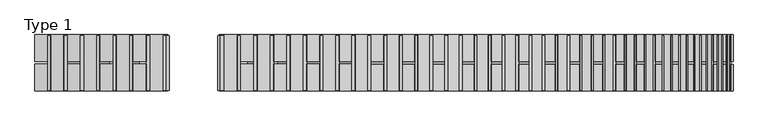
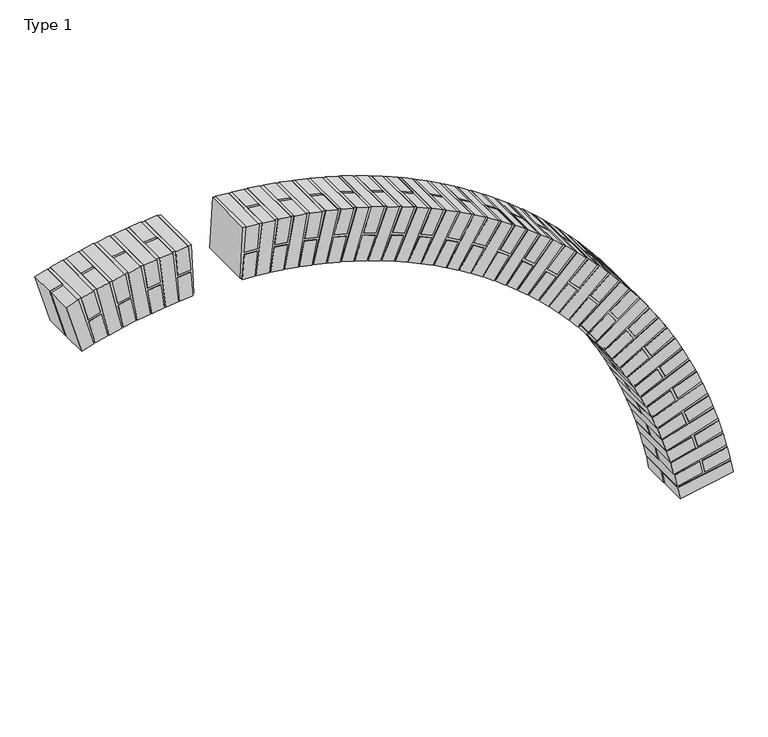
"""IFC4 building model written with IfcOpenShell, lengths in millimetres: proxy geometry, 00_GM_toog : Type 1."""

from ifc_helpers import new_model, si_unit, frame, origin, place, context, project, spatial, polyline, outline, extrude, source, transform, mapped, element, save


def type_1_09ec10ce(model_context):
    return source(origin(), model_context, "Body", "SweptSolid", [
        extrude(outline(polyline([(-51.3105527, 298.3168038), (-50.0324743, 286.1851231), (-149.0433825, 272.1551526), (-142.0283972, 222.6496985), (-43.0174891, 236.6796691), (-41.3072329, 224.6102198), (-244.0930868, 202.1502071), (-245.111966, 208.0426268), (-151.9800205, 221.2395409), (-158.9950058, 270.744995), (-252.3004379, 257.5234976), (-253.31442, 263.3875962), (-51.3105527, 298.3168038)])), frame((0.0, 2.5, 0.0), z_axis=(0.0, 1.0, 0.0), x_axis=(0.0, 0.0, 1.0)), (0.0, 0.0, 1.0), 205.0),
        extrude(outline(polyline([(0.0, 50.0), (210.0, 50.0), (210.0, 0.0), (0.0, 0.0), (0.0, 50.0)])), frame((222.6496985, 210.0, -142.0283972), z_axis=(0.14029970561810096, 0.0, 0.9901090811640273), x_axis=(0.0, -1.0, 0.0)), (0.0, 0.0, 1.0), 100.0),
        extrude(outline(polyline([(0.0, 49.9999999), (210.0, 49.9999999), (210.0, 0.0), (0.0, 0.0), (0.0, 49.9999999)])), frame((207.2095704, 210.0, -250.9909286), z_axis=(0.14029970561810096, 0.0, 0.9901090811640273), x_axis=(0.0, -1.0, 0.0)), (0.0, 0.0, 1.0), 100.0),
        extrude(outline(polyline([(210.0, 50.0), (210.0, 0.0), (110.0, 0.0), (110.0, 50.0), (210.0, 50.0)])), frame((311.8048021, 0.0, -266.7590939), z_axis=(0.17038513774279196, 0.0, 0.9853775443130262), x_axis=(0.0, 1.0, 0.0)), (0.0, 0.0, 1.0), 210.0),
        extrude(outline(polyline([(100.0, 50.0), (100.0, 0.0), (0.0, 0.0), (0.0, 50.0), (100.0, 50.0)])), frame((311.8048021, 0.0, -266.7590939), z_axis=(0.17038513774279196, 0.0, 0.9853775443130262), x_axis=(0.0, 1.0, 0.0)), (0.0, 0.0, 1.0), 210.0),
        extrude(outline(polyline([(-36.8943593, 174.8755374), (-36.357169, 162.6885531), (-136.0385268, 154.7119056), (-132.0502031, 104.8712267), (-32.3688453, 112.8478742), (-31.3964904, 100.696697), (-235.1735118, 90.6229563), (-235.8317995, 96.5664722), (-142.0692136, 104.0694909), (-146.0575373, 153.9101698), (-239.9947846, 146.3931745), (-240.6499084, 152.3081238), (-36.8943593, 174.8755374)])), frame((0.0, 2.5, 0.0), z_axis=(0.0, 1.0, 0.0), x_axis=(0.0, 0.0, 1.0)), (0.0, 0.0, 1.0), 205.0),
        extrude(outline(polyline([(0.0, 50.0), (210.0, 50.0), (210.0, 0.0), (0.0, 0.0), (0.0, 50.0)])), frame((104.8712267, 210.0, -132.0502031), z_axis=(0.07976647429823253, 0.0, 0.9968135781469017), x_axis=(0.0, -1.0, 0.0)), (0.0, 0.0, 1.0), 100.0),
        extrude(outline(polyline([(0.0, 50.0), (210.0, 50.0), (210.0, 0.0), (0.0, 0.0), (0.0, 50.0)])), frame((96.0928435, 210.0, -241.7505714), z_axis=(0.07976647429823253, 0.0, 0.9968135781469017), x_axis=(0.0, -1.0, 0.0)), (0.0, 0.0, 1.0), 100.0),
        extrude(outline(polyline([(210.0, 50.0), (210.0, 0.0), (110.0, 0.0), (110.0, 50.0), (210.0, 50.0)])), frame((201.453981, 0.0, -251.1222434), z_axis=(0.11008414261687069, 0.0, 0.9939222713795623), x_axis=(0.0, 1.0, 0.0)), (0.0, 0.0, 1.0), 210.0),
        extrude(outline(polyline([(100.0, 50.0), (100.0, 0.0), (0.0, 0.0), (0.0, 50.0), (100.0, 50.0)])), frame((201.453981, 0.0, -251.1222434), z_axis=(0.11008414261687069, 0.0, 0.9939222713795623), x_axis=(0.0, 1.0, 0.0)), (0.0, 0.0, 1.0), 210.0),
        extrude(outline(polyline([(-73.2145142, 420.6515468), (-71.2002884, 408.6201689), (-169.1734934, 388.5889155), (-159.1578667, 339.602313), (-61.1846617, 359.6335665), (-58.742848, 347.6906134), (-259.7853565, 312.9276379), (-261.161048, 318.747105), (-169.0051901, 337.5889643), (-179.0208168, 386.5755668), (-271.348343, 367.6986088), (-272.7174225, 373.4901055), (-73.2145142, 420.6515468)])), frame((0.0, 2.5, 0.0), z_axis=(0.0, 1.0, 0.0), x_axis=(0.0, 0.0, 1.0)), (0.0, 0.0, 1.0), 205.0),
        extrude(outline(polyline([(0.0, 50.0), (210.0, 50.0), (210.0, 0.0), (0.0, 0.0), (0.0, 50.0)])), frame((339.602313, 210.0, -159.1578667), z_axis=(0.20031253413085065, 0.0, 0.9797320494247787), x_axis=(0.0, -1.0, 0.0)), (0.0, 0.0, 1.0), 100.0),
        extrude(outline(polyline([(0.0, 49.9999999), (210.0, 49.9999999), (210.0, 0.0), (0.0, 0.0), (0.0, 49.9999999)])), frame((317.5577109, 210.0, -266.978395), z_axis=(0.20031253413085065, 0.0, 0.9797320494247787), x_axis=(0.0, -1.0, 0.0)), (0.0, 0.0, 1.0), 100.0),
        extrude(outline(polyline([(210.0, 50.0), (210.0, 0.0), (110.0, 0.0), (110.0, 50.0), (210.0, 50.0)])), frame((420.9990698, 0.0, -289.084566), z_axis=(0.2300541365036329, 0.0, 0.973177832812466), x_axis=(0.0, 1.0, 0.0)), (0.0, 0.0, 1.0), 210.0),
        extrude(outline(polyline([(100.0, 50.0), (100.0, 0.0), (0.0, 0.0), (0.0, 50.0), (100.0, 50.0)])), frame((420.9990698, 0.0, -289.084566), z_axis=(0.2300541365036329, 0.0, 0.973177832812466), x_axis=(0.0, 1.0, 0.0)), (0.0, 0.0, 1.0), 210.0),
        extrude(outline(polyline([(-102.5249972, 541.4259997), (-99.7820951, 529.5395517), (-196.3541925, 503.5813158), (-183.3750746, 455.2952671), (-86.8029772, 481.253503), (-83.6386631, 469.4813452), (-282.1921149, 422.5443504), (-283.9195159, 428.2692793), (-193.0815721, 452.6861951), (-206.06069, 500.9722438), (-297.0678472, 476.509844), (-298.7869457, 482.2072569), (-102.5249972, 541.4259997)])), frame((0.0, 2.5, 0.0), z_axis=(0.0, 1.0, 0.0), x_axis=(0.0, 0.0, 1.0)), (0.0, 0.0, 1.0), 205.0),
        extrude(outline(polyline([(0.0, 50.0), (210.0, 50.0), (210.0, 0.0), (0.0, 0.0), (0.0, 50.0)])), frame((455.2952671, 210.0, -183.3750746), z_axis=(0.2595823589102464, 0.0, 0.9657209736474569), x_axis=(0.0, -1.0, 0.0)), (0.0, 0.0, 1.0), 100.0),
        extrude(outline(polyline([(0.0, 50.0), (210.0, 50.0), (210.0, 0.0), (0.0, 0.0), (0.0, 50.0)])), frame((426.7279592, 210.0, -289.6536695), z_axis=(0.2595823589102464, 0.0, 0.9657209736474569), x_axis=(0.0, -1.0, 0.0)), (0.0, 0.0, 1.0), 100.0),
        extrude(outline(polyline([(210.0, 50.0000001), (210.0, 0.0), (110.0, 0.0), (110.0, 50.0000001), (210.0, 50.0000001)])), frame((528.6317584, 0.0, -318.0158494), z_axis=(0.28886981331416434, 0.0, 0.9573683883207341), x_axis=(0.0, 1.0, 0.0)), (0.0, 0.0, 1.0), 210.0),
        extrude(outline(polyline([(100.0, 50.0000001), (100.0, 0.0), (0.0, 0.0), (0.0, 50.0000001), (100.0, 50.0000001)])), frame((528.6317584, 0.0, -318.0158494), z_axis=(0.28886981331416434, 0.0, 0.9573683883207341), x_axis=(0.0, 1.0, 0.0)), (0.0, 0.0, 1.0), 210.0),
        extrude(outline(polyline([(-139.1332824, 660.1921832), (-135.6718782, 648.4947544), (-230.4846606, 616.7058209), (-214.5901938, 569.2994297), (-119.7774114, 601.0883632), (-115.9023342, 589.5306663), (-311.2302503, 530.593752), (-313.3029535, 536.2029076), (-224.119862, 566.1043122), (-240.0143287, 613.5107034), (-329.3635509, 583.5535983), (-331.426292, 589.1357943), (-139.1332824, 660.1921832)])), frame((0.0, 2.5, 0.0), z_axis=(0.0, 1.0, 0.0), x_axis=(0.0, 0.0, 1.0)), (0.0, 0.0, 1.0), 205.0),
        extrude(outline(polyline([(0.0, 50.0), (210.0, 50.0), (210.0, 0.0), (0.0, 0.0), (0.0, 50.0)])), frame((569.2994297, 210.0, -214.5901938), z_axis=(0.3178893349961213, 0.0, 0.9481278240278174), x_axis=(0.0, -1.0, 0.0)), (0.0, 0.0, 1.0), 100.0),
        extrude(outline(polyline([(0.0, 50.0), (210.0, 50.0), (210.0, 0.0), (0.0, 0.0), (0.0, 50.0)])), frame((534.3153787, 210.0, -318.9326444), z_axis=(0.3178893349961213, 0.0, 0.9481278240278174), x_axis=(0.0, -1.0, 0.0)), (0.0, 0.0, 1.0), 100.0),
        extrude(outline(polyline([(210.0, 50.0), (210.0, 0.0), (110.0, 0.0), (110.0, 50.0), (210.0, 50.0)])), frame((634.3036342, 0.0, -353.4456316), z_axis=(0.3466140077500296, 0.0, 0.9380078515830571), x_axis=(0.0, 1.0, 0.0)), (0.0, 0.0, 1.0), 210.0),
        extrude(outline(polyline([(100.0, 50.0), (100.0, 0.0), (0.0, 0.0), (0.0, 50.0), (100.0, 50.0)])), frame((634.3036342, 0.0, -353.4456316), z_axis=(0.3466140077500296, 0.0, 0.9380078515830571), x_axis=(0.0, 1.0, 0.0)), (0.0, 0.0, 1.0), 210.0),
        extrude(outline(polyline([(-182.9035816, 776.5095671), (-178.7365144, 765.0445459), (-271.4383001, 727.5428271), (-252.6874407, 681.1919342), (-159.9856549, 718.6936531), (-155.414188, 707.3932871), (-346.7920539, 636.6750634), (-349.2023711, 642.14764), (-262.0049317, 677.4226224), (-280.7557912, 723.7735153), (-368.1156623, 688.4328225), (-370.5143948, 693.8790961), (-182.9035816, 776.5095671)])), frame((0.0, 2.5, 0.0), z_axis=(0.0, 1.0, 0.0), x_axis=(0.0, 0.0, 1.0)), (0.0, 0.0, 1.0), 205.0),
        extrude(outline(polyline([(0.0, 50.0), (210.0, 50.0), (210.0, 0.0), (0.0, 0.0), (0.0, 50.0)])), frame((681.1919342, 210.0, -252.6874407), z_axis=(0.37501718884823365, 0.0, 0.9270178574700534), x_axis=(0.0, -1.0, 0.0)), (0.0, 0.0, 1.0), 100.0),
        extrude(outline(polyline([(0.0, 50.0), (210.0, 50.0), (210.0, 0.0), (0.0, 0.0), (0.0, 50.0)])), frame((639.9209035, 210.0, -354.7067175), z_axis=(0.37501718884823365, 0.0, 0.9270178574700534), x_axis=(0.0, -1.0, 0.0)), (0.0, 0.0, 1.0), 100.0),
        extrude(outline(polyline([(210.0, 50.0), (210.0, 0.0), (110.0, 0.0), (110.0, 50.0), (210.0, 50.0)])), frame((737.6227368, 0.0, -395.2424957), z_axis=(0.40307253375327073, 0.0, 0.9151680351354708), x_axis=(0.0, 1.0, 0.0)), (0.0, 0.0, 1.0), 210.0),
        extrude(outline(polyline([(100.0, 50.0), (100.0, 0.0), (0.0, 0.0), (0.0, 50.0), (100.0, 50.0)])), frame((737.6227368, 0.0, -395.2424957), z_axis=(0.40307253375327073, 0.0, 0.9151680351354708), x_axis=(0.0, 1.0, 0.0)), (0.0, 0.0, 1.0), 210.0),
        extrude(outline(polyline([(-233.6735411, 889.9467043), (-228.8162674, 878.7566171), (-319.0632049, 835.6812151), (-297.5255039, 790.5577463), (-207.2785664, 833.6331483), (-202.0276663, 822.6320289), (-388.7456188, 740.3948054), (-391.4846098, 745.7105041), (-306.5962573, 786.2282216), (-328.1339583, 831.3516903), (-413.1804412, 790.7584963), (-415.9062676, 796.048646), (-233.6735411, 889.9467043)])), frame((0.0, 2.5, 0.0), z_axis=(0.0, 1.0, 0.0), x_axis=(0.0, 0.0, 1.0)), (0.0, 0.0, 1.0), 205.0),
        extrude(outline(polyline([(0.0, 50.0), (210.0, 50.0), (210.0, 0.0), (0.0, 0.0), (0.0, 50.0)])), frame((790.5577463, 210.0, -297.5255039), z_axis=(0.43075402055290246, 0.0, 0.9024693755344331), x_axis=(0.0, -1.0, 0.0)), (0.0, 0.0, 1.0), 100.0),
        extrude(outline(polyline([(0.0, 50.0), (210.0, 50.0), (210.0, 0.0), (0.0, 0.0), (0.0, 50.0)])), frame((743.1528195, 210.0, -396.8431948), z_axis=(0.43075402055290246, 0.0, 0.9024693755344331), x_axis=(0.0, -1.0, 0.0)), (0.0, 0.0, 1.0), 100.0),
        extrude(outline(polyline([(210.0, 50.0), (210.0, 0.0), (110.0, 0.0), (110.0, 50.0), (210.0, 50.0)])), frame((838.2058326, 0.0, -443.2514078), z_axis=(0.458035974096042, 0.0, 0.8889336569361574), x_axis=(0.0, 1.0, 0.0)), (0.0, 0.0, 1.0), 210.0),
        extrude(outline(polyline([(100.0, 50.0), (100.0, 0.0), (0.0, 0.0), (0.0, 50.0), (100.0, 50.0)])), frame((838.2058326, 0.0, -443.2514078), z_axis=(0.458035974096042, 0.0, 0.8889336569361574), x_axis=(0.0, 1.0, 0.0)), (0.0, 0.0, 1.0), 210.0),
        extrude(outline(polyline([(-291.2548438, 1000.0828313), (-285.7253803, 989.2091846), (-373.1827237, 940.7198756), (-348.9380692, 896.9912039), (-261.4807258, 945.4805129), (-255.5698695, 934.8194455), (-436.9353302, 841.3682584), (-439.9928353, 846.5073621), (-357.7284394, 892.1175254), (-381.9730939, 935.8461971), (-464.3907322, 890.151071), (-467.4335419, 895.2654744), (-291.2548438, 1000.0828313)])), frame((0.0, 2.5, 0.0), z_axis=(0.0, 1.0, 0.0), x_axis=(0.0, 0.0, 1.0)), (0.0, 0.0, 1.0), 205.0),
        extrude(outline(polyline([(0.0, 50.0), (210.0, 50.0), (210.0, 0.0), (0.0, 0.0), (0.0, 50.0)])), frame((896.9912039, 210.0, -348.9380692), z_axis=(0.4848930898069246, 0.0, 0.8745734339993948), x_axis=(0.0, -1.0, 0.0)), (0.0, 0.0, 1.0), 100.0),
        extrude(outline(polyline([(0.0, 50.0), (210.0, 50.0), (210.0, 0.0), (0.0, 0.0), (0.0, 50.0)])), frame((843.6282164, 210.0, -445.1857828), z_axis=(0.4848930898069246, 0.0, 0.8745734339993948), x_axis=(0.0, -1.0, 0.0)), (0.0, 0.0, 1.0), 100.0),
        extrude(outline(polyline([(210.0, 50.0), (210.0, 0.0), (110.0, 0.0), (110.0, 50.0), (210.0, 50.0)])), frame((935.6798366, 0.0, -497.2942922), z_axis=(0.5113004571556836, 0.0, 0.8594020261276959), x_axis=(0.0, 1.0, 0.0)), (0.0, 0.0, 1.0), 210.0),
        extrude(outline(polyline([(100.0, 50.0), (100.0, 0.0), (0.0, 0.0), (0.0, 50.0), (100.0, 50.0)])), frame((935.6798366, 0.0, -497.2942922), z_axis=(0.5113004571556836, 0.0, 0.8594020261276959), x_axis=(0.0, 1.0, 0.0)), (0.0, 0.0, 1.0), 210.0),
        extrude(outline(polyline([(-355.4339079, 1106.5094287), (-349.2527645, 1095.9925552), (-433.5961151, 1042.2691969), (-406.7344359, 1000.0975217), (-322.3910854, 1053.82088), (-315.8421974, 1043.5394089), (-491.1824416, 939.2208894), (-494.5471198, 944.1643361), (-415.2118175, 994.6977669), (-442.0734967, 1036.8694422), (-521.5565851, 986.2418775), (-524.9050916, 991.1615642), (-355.4339079, 1106.5094287)])), frame((0.0, 2.5, 0.0), z_axis=(0.0, 1.0, 0.0), x_axis=(0.0, 0.0, 1.0)), (0.0, 0.0, 1.0), 205.0),
        extrude(outline(polyline([(0.0, 50.0), (210.0, 50.0), (210.0, 0.0), (0.0, 0.0), (0.0, 50.0)])), frame((1000.0975217, 210.0, -406.7344359), z_axis=(0.5372335827633249, 0.0, 0.8434335051154191), x_axis=(0.0, -1.0, 0.0)), (0.0, 0.0, 1.0), 100.0),
        extrude(outline(polyline([(0.0, 50.0), (210.0, 50.0), (210.0, 0.0), (0.0, 0.0), (0.0, 50.0)])), frame((940.9744086, 210.0, -499.5551681), z_axis=(0.5372335827633249, 0.0, 0.8434335051154191), x_axis=(0.0, -1.0, 0.0)), (0.0, 0.0, 1.0), 100.0),
        extrude(outline(polyline([(210.0, 50.0), (210.0, 0.0), (110.0, 0.0), (110.0, 50.0), (210.0, 50.0)])), frame((1029.683196, 0.0, -557.1706918), z_axis=(0.562668413119899, 0.0, 0.8266826820958176), x_axis=(0.0, 1.0, 0.0)), (0.0, 0.0, 1.0), 210.0),
        extrude(outline(polyline([(100.0, 50.0), (100.0, 0.0), (0.0, 0.0), (0.0, 50.0), (100.0, 50.0)])), frame((1029.683196, 0.0, -557.1706918), z_axis=(0.562668413119899, 0.0, 0.8266826820958176), x_axis=(0.0, 1.0, 0.0)), (0.0, 0.0, 1.0), 210.0),
        extrude(outline(polyline([(-425.9726788, 1208.8317365), (-419.162783, 1198.7106457), (-500.0792923, 1139.9525101), (-470.7002245, 1099.4942554), (-389.7837151, 1158.252391), (-382.6210868, 1148.3886526), (-551.2857383, 1033.5897414), (-554.9451095, 1038.3191945), (-478.833173, 1093.5884532), (-508.2122409, 1134.0467079), (-584.4659589, 1078.6744934), (-588.1077418, 1083.3812152), (-425.9726788, 1208.8317365)])), frame((0.0, 2.5, 0.0), z_axis=(0.0, 1.0, 0.0), x_axis=(0.0, 0.0, 1.0)), (0.0, 0.0, 1.0), 205.0),
        extrude(outline(polyline([(0.0, 50.0), (210.0, 50.0), (210.0, 0.0), (0.0, 0.0), (0.0, 50.0)])), frame((1099.4942554, 210.0, -470.7002245), z_axis=(0.587581356894572, 0.0, 0.8091650938034423), x_axis=(0.0, -1.0, 0.0)), (0.0, 0.0, 1.0), 100.0),
        extrude(outline(polyline([(0.0, 50.0), (210.0, 50.0), (210.0, 0.0), (0.0, 0.0), (0.0, 50.0)])), frame((1034.8303175, 210.0, -559.7496824), z_axis=(0.587581356894572, 0.0, 0.8091650938034423), x_axis=(0.0, -1.0, 0.0)), (0.0, 0.0, 1.0), 100.0),
        extrude(outline(polyline([(210.0, 50.0), (210.0, 0.0), (110.0, 0.0), (110.0, 50.0), (210.0, 50.0)])), frame((1119.8672315, 0.0, -622.6585117), z_axis=(0.6119493068171298, 0.0, 0.7908969881634614), x_axis=(0.0, 1.0, 0.0)), (0.0, 0.0, 1.0), 210.0),
        extrude(outline(polyline([(100.0, 50.0), (100.0, 0.0), (0.0, 0.0), (0.0, 50.0), (100.0, 50.0)])), frame((1119.8672315, 0.0, -622.6585117), z_axis=(0.6119493068171298, 0.0, 0.7908969881634614), x_axis=(0.0, 1.0, 0.0)), (0.0, 0.0, 1.0), 210.0),
        extrude(outline(polyline([(-502.6095127, 1306.6702186), (-495.1961237, 1296.9824519), (-572.3856546, 1233.4074858), (-540.5981716, 1194.8127203), (-463.4086406, 1258.3876865), (-455.6588397, 1248.9782674), (-617.022284, 1124.1247791), (-620.9627746, 1128.6226962), (-548.3565201, 1188.4227768), (-580.1440032, 1227.0175422), (-652.8855088, 1167.1060659), (-656.80706, 1171.5823645), (-502.6095127, 1306.6702186)])), frame((0.0, 2.5, 0.0), z_axis=(0.0, 1.0, 0.0), x_axis=(0.0, 0.0, 1.0)), (0.0, 0.0, 1.0), 205.0),
        extrude(outline(polyline([(0.0, 50.0), (210.0, 50.0), (210.0, 0.0), (0.0, 0.0), (0.0, 50.0)])), frame((1194.8127203, 210.0, -540.5981716), z_axis=(0.6357496611103878, 0.0, 0.771895309221417), x_axis=(0.0, -1.0, 0.0)), (0.0, 0.0, 1.0), 100.0),
        extrude(outline(polyline([(0.0, 50.0), (210.0, 50.0), (210.0, 0.0), (0.0, 0.0), (0.0, 50.0)])), frame((1124.8478107, 210.0, -625.546051), z_axis=(0.6357496611103878, 0.0, 0.771895309221417), x_axis=(0.0, -1.0, 0.0)), (0.0, 0.0, 1.0), 100.0),
        extrude(outline(polyline([(210.0, 50.0), (210.0, 0.0), (110.0, 0.0), (110.0, 50.0), (210.0, 50.0)])), frame((1205.8974304, 0.0, -693.514843), z_axis=(0.658960344453872, 0.0, 0.752177681427224), x_axis=(0.0, 1.0, 0.0)), (0.0, 0.0, 1.0), 210.0),
        extrude(outline(polyline([(100.0, 50.0), (100.0, 0.0), (0.0, 0.0), (0.0, 50.0), (100.0, 50.0)])), frame((1205.8974304, 0.0, -693.514843), z_axis=(0.658960344453872, 0.0, 0.752177681427224), x_axis=(0.0, 1.0, 0.0)), (0.0, 0.0, 1.0), 210.0),
        extrude(outline(polyline([(-585.0601464, 1399.6619703), (-577.0707622, 1390.4434618), (-650.2470015, 1322.2874789), (-616.1690101, 1285.6993592), (-542.9927708, 1353.8553421), (-534.684543, 1344.9351441), (-688.1482472, 1210.490188), (-692.355241, 1214.7398854), (-623.5239812, 1278.848976), (-657.6019727, 1315.4370957), (-726.5614515, 1251.2085824), (-730.7482251, 1255.4378542), (-585.0601464, 1399.6619703)])), frame((0.0, 2.5, 0.0), z_axis=(0.0, 1.0, 0.0), x_axis=(0.0, 0.0, 1.0)), (0.0, 0.0, 1.0), 205.0),
        extrude(outline(polyline([(0.0, 50.0), (210.0, 50.0), (210.0, 0.0), (0.0, 0.0), (0.0, 50.0)])), frame((1285.6993592, 210.0, -616.1690101), z_axis=(0.6815598284590672, 0.0, 0.7317623932881814), x_axis=(0.0, -1.0, 0.0)), (0.0, 0.0, 1.0), 100.0),
        extrude(outline(polyline([(0.0, 50.0), (210.0, 50.0), (210.0, 0.0), (0.0, 0.0), (0.0, 50.0)])), frame((1210.6929931, 210.0, -696.7002206), z_axis=(0.6815598284590672, 0.0, 0.7317623932881814), x_axis=(0.0, -1.0, 0.0)), (0.0, 0.0, 1.0), 100.0),
        extrude(outline(polyline([(210.0, 50.0), (210.0, 0.0), (110.0, 0.0), (110.0, 50.0), (210.0, 50.0)])), frame((1287.4546875, 0.0, -769.4768639), z_axis=(0.7035271516375073, 0.0, 0.7106683804059498), x_axis=(0.0, 1.0, 0.0)), (0.0, 0.0, 1.0), 210.0),
        extrude(outline(polyline([(100.0, 50.0), (100.0, 0.0), (0.0, 0.0), (0.0, 50.0), (100.0, 50.0)])), frame((1287.4546875, 0.0, -769.4768639), z_axis=(0.7035271516375073, 0.0, 0.7106683804059498), x_axis=(0.0, 1.0, 0.0)), (0.0, 0.0, 1.0), 210.0),
        extrude(outline(polyline([(-673.0187522, 1487.4620645), (-664.4830073, 1478.7470076), (-733.374528, 1406.2628137), (-697.1324311, 1371.8170533), (-628.2409103, 1444.3012472), (-619.4050728, 1435.9033572), (-764.3998058, 1292.3656196), (-768.8576982, 1296.3513341), (-704.0567436, 1364.53164), (-740.2988405, 1398.9774004), (-805.2205066, 1330.670088), (-809.6569728, 1334.6366457), (-673.0187522, 1487.4620645)])), frame((0.0, 2.5, 0.0), z_axis=(0.0, 1.0, 0.0), x_axis=(0.0, 0.0, 1.0)), (0.0, 0.0, 1.0), 205.0),
        extrude(outline(polyline([(0.0, 99.9999999), (210.0, 99.9999999), (210.0, 0.0), (0.0, 0.0), (0.0, 99.9999999)])), frame((1406.2628137, 210.0, -733.374528), z_axis=(-0.6889152079134424, 0.0, 0.7248419388429304), x_axis=(0.0, -1.0, 0.0)), (0.0, 0.0, 1.0), 50.0),
        extrude(outline(polyline([(0.0, 100.0), (210.0, 100.0), (210.0, 0.0), (0.0, 0.0), (0.0, 100.0)])), frame((1326.4932065, 210.0, -809.1903613), z_axis=(-0.6889152079134424, 0.0, 0.7248419388429304), x_axis=(0.0, -1.0, 0.0)), (0.0, 0.0, 1.0), 50.0),
        extrude(outline(polyline([(0.0, 100.0), (209.9999999, 100.0), (209.9999999, 0.0), (0.0, 0.0), (0.0, 100.0)])), frame((1364.2364889, 110.0, -850.2628142), z_axis=(-0.6665230523277088, 0.0, 0.7454844201697004), x_axis=(0.7454844201697004, 0.0, 0.6665230523277088)), (0.0, 0.0, 1.0), 50.0),
        extrude(outline(polyline([(0.0, 100.0), (209.9999999, 100.0), (209.9999999, 0.0), (0.0, 0.0), (0.0, 100.0)])), frame((1364.2364889, 0.0, -850.2628142), z_axis=(-0.6665230523277088, 0.0, 0.7454844201697004), x_axis=(0.7454844201697004, 0.0, 0.6665230523277088)), (0.0, 0.0, 1.0), 50.0),
        extrude(outline(polyline([(-766.1590722, 1569.7448312), (-757.1086274, 1561.565552), (-821.4598957, 1485.022007), (-783.1881232, 1452.8463729), (-718.8368549, 1529.3899178), (-709.5061817, 1521.5454855), (-845.4941258, 1369.4473798), (-850.1863815, 1373.1543275), (-789.6560932, 1445.1529526), (-827.9278656, 1477.3285868), (-888.57091, 1405.1958423), (-893.2406131, 1408.8849732), (-766.1590722, 1569.7448312)])), frame((0.0, 2.5, 0.0), z_axis=(0.0, 1.0, 0.0), x_axis=(0.0, 0.0, 1.0)), (0.0, 0.0, 1.0), 205.0),
        extrude(outline(polyline([(0.0, 100.0000001), (210.0, 100.0000001), (210.0, 0.0), (0.0, 0.0), (0.0, 100.0000001)])), frame((1485.022007, 210.0, -821.4598957), z_axis=(-0.643512682835849, 0.0, 0.7654354492897545), x_axis=(0.0, -1.0, 0.0)), (0.0, 0.0, 1.0), 50.0),
        extrude(outline(polyline([(0.0, 100.0), (210.0, 100.0), (210.0, 0.0), (0.0, 0.0), (0.0, 100.0)])), frame((1400.7850419, 210.0, -892.2791339), z_axis=(-0.643512682835849, 0.0, 0.7654354492897545), x_axis=(0.0, -1.0, 0.0)), (0.0, 0.0, 1.0), 50.0),
        extrude(outline(polyline([(0.0, 100.0), (210.0, 100.0), (210.0, 0.0), (0.0, 0.0), (0.0, 100.0)])), frame((1435.9580338, 110.0, -935.5730411), z_axis=(-0.6199054420311093, 0.0, 0.7846765212112665), x_axis=(0.7846765212112665, 0.0, 0.6199054420311093)), (0.0, 0.0, 1.0), 50.0),
        extrude(outline(polyline([(0.0, 100.0), (210.0, 100.0), (210.0, 0.0), (0.0, 0.0), (0.0, 100.0)])), frame((1435.9580338, 0.0, -935.5730411), z_axis=(-0.6199054420311093, 0.0, 0.7846765212112665), x_axis=(0.7846765212112665, 0.0, 0.6199054420311093)), (0.0, 0.0, 1.0), 50.0),
        extrude(outline(polyline([(-864.1356281, 1646.2050652), (-854.6040536, 1638.5919024), (-914.1763762, 1558.2729235), (-874.0168867, 1528.4867622), (-814.4445641, 1608.8057411), (-804.6536647, 1601.5438633), (-931.1304104, 1441.4495551), (-936.0396247, 1444.8639862), (-880.0045231, 1520.4138717), (-920.1640125, 1550.200033), (-976.3034966, 1474.5094128), (-981.1891156, 1477.9074329), (-864.1356281, 1646.2050652)])), frame((0.0, 2.5, 0.0), z_axis=(0.0, 1.0, 0.0), x_axis=(0.0, 0.0, 1.0)), (0.0, 0.0, 1.0), 205.0),
        extrude(outline(polyline([(0.0, 100.0), (210.0, 100.0), (210.0, 0.0), (0.0, 0.0), (0.0, 100.0)])), frame((1558.2729235, 210.0, -914.1763762), z_axis=(-0.5957232261172445, 0.0, 0.8031897894423599), x_axis=(0.0, -1.0, 0.0)), (0.0, 0.0, 1.0), 50.0),
        extrude(outline(polyline([(0.0, 100.0), (210.0, 100.0), (210.0, 0.0), (0.0, 0.0), (0.0, 100.0)])), frame((1469.881054, 210.0, -979.7363351), z_axis=(-0.5957232261172445, 0.0, 0.8031897894423599), x_axis=(0.0, -1.0, 0.0)), (0.0, 0.0, 1.0), 50.0),
        extrude(outline(polyline([(0.0, 100.0), (210.0, 100.0), (210.0, 0.0), (0.0, 0.0), (0.0, 100.0)])), frame((1502.3532911, 110.0, -1025.0911098), z_axis=(-0.5709884645992758, 0.0, 0.8209580825441465), x_axis=(0.8209580825441465, 0.0, 0.5709884645992758)), (0.0, 0.0, 1.0), 50.0),
        extrude(outline(polyline([(0.0, 100.0), (210.0, 100.0), (210.0, 0.0), (0.0, 0.0), (0.0, 100.0)])), frame((1502.3532911, 0.0, -1025.0911098), z_axis=(-0.5709884645992758, 0.0, 0.8209580825441465), x_axis=(0.8209580825441465, 0.0, 0.5709884645992758)), (0.0, 0.0, 1.0), 50.0),
        extrude(outline(polyline([(-966.5850031, 1716.5591585), (-956.6076536, 1709.5403512), (-1011.1800635, 1625.7438592), (-969.2818175, 1598.4576542), (-914.7094076, 1682.2541462), (-904.4945987, 1675.6017587), (-1020.9910156, 1508.1050735), (-1026.0989792, 1511.214323), (-974.7669108, 1590.0352375), (-1016.6651568, 1617.3214425), (-1068.0928468, 1538.3537), (-1073.1762598, 1541.4480054), (-966.5850031, 1716.5591585)])), frame((0.0, 2.5, 0.0), z_axis=(0.0, 1.0, 0.0), x_axis=(0.0, 0.0, 1.0)), (0.0, 0.0, 1.0), 205.0),
        extrude(outline(polyline([(0.0, 100.0), (210.0, 100.0), (210.0, 0.0), (0.0, 0.0), (0.0, 100.0)])), frame((1625.7438592, 210.0, -1011.1800635), z_axis=(-0.5457240994797231, 0.0, 0.8379649200575435), x_axis=(0.0, -1.0, 0.0)), (0.0, 0.0, 1.0), 50.0),
        extrude(outline(polyline([(0.0, 100.0), (210.0, 100.0), (210.0, 0.0), (0.0, 0.0), (0.0, 100.0)])), frame((1533.5249505, 210.0, -1071.2375667), z_axis=(-0.5457240994797231, 0.0, 0.8379649200575435), x_axis=(0.0, -1.0, 0.0)), (0.0, 0.0, 1.0), 50.0),
        extrude(outline(polyline([(0.0, 100.0), (210.0, 100.0), (210.0, 0.0), (0.0, 0.0), (0.0, 100.0)])), frame((1563.1759859, 110.0, -1118.4849779), z_axis=(-0.5199535639793587, 0.0, 0.854194527789287), x_axis=(0.854194527789287, 0.0, 0.5199535639793587)), (0.0, 0.0, 1.0), 50.0),
        extrude(outline(polyline([(0.0, 100.0), (210.0, 100.0), (210.0, 0.0), (0.0, 0.0), (0.0, 100.0)])), frame((1563.1759859, 0.0, -1118.4849779), z_axis=(-0.5199535639793587, 0.0, 0.854194527789287), x_axis=(0.854194527789287, 0.0, 0.5199535639793587)), (0.0, 0.0, 1.0), 50.0),
        extrude(outline(polyline([(-1073.1271897, 1780.5461522), (-1062.7410734, 1774.1477346), (-1112.1111495, 1687.1845493), (-1068.6295568, 1662.4995113), (-1019.2594808, 1749.4626965), (-1008.6586513, 1743.4444745), (-1114.7426284, 1569.1666948), (-1120.0303947, 1571.9592298), (-1073.5917616, 1653.7588091), (-1117.0733542, 1678.4438472), (-1163.5984934, 1596.4918913), (-1168.8608449, 1599.2710044), (-1073.1271897, 1780.5461522)])), frame((0.0, 2.5, 0.0), z_axis=(0.0, 1.0, 0.0), x_axis=(0.0, 0.0, 1.0)), (0.0, 0.0, 1.0), 205.0),
        extrude(outline(polyline([(0.0, 100.0000001), (210.0, 100.0000001), (210.0, 0.0), (0.0, 0.0), (0.0, 100.0000001)])), frame((1687.1845493, 210.0, -1112.1111495), z_axis=(-0.4937007608024789, 0.0, 0.8696318524427756), x_axis=(0.0, -1.0, 0.0)), (0.0, 0.0, 1.0), 50.0),
        extrude(outline(polyline([(0.0, 100.0000001), (210.0, 100.0000001), (210.0, 0.0), (0.0, 0.0), (0.0, 100.0000001)])), frame((1591.4806619, 210.0, -1166.4434303), z_axis=(-0.4937007608024789, 0.0, 0.8696318524427756), x_axis=(0.0, -1.0, 0.0)), (0.0, 0.0, 1.0), 50.0),
        extrude(outline(polyline([(0.0, 100.0), (210.0, 100.0), (210.0, 0.0), (0.0, 0.0), (0.0, 100.0)])), frame((1618.2005133, 110.0, -1215.4082269), z_axis=(-0.46699003996658267, 0.0, 0.8842625755803587), x_axis=(0.8842625755803587, 0.0, 0.46699003996658267)), (0.0, 0.0, 1.0), 50.0),
        extrude(outline(polyline([(0.0, 100.0), (210.0, 100.0), (210.0, 0.0), (0.0, 0.0), (0.0, 100.0)])), frame((1618.2005133, 0.0, -1215.4082269), z_axis=(-0.46699003996658267, 0.0, 0.8842625755803587), x_axis=(0.8842625755803587, 0.0, 0.46699003996658267)), (0.0, 0.0, 1.0), 50.0),
        extrude(outline(polyline([(-1183.3669992, 1837.9287043), (-1172.6106405, 1832.1744095), (-1216.5952582, 1742.3670968), (-1171.6916018, 1720.374788), (-1127.7069842, 1810.1821007), (-1116.7594551, 1804.8203672), (-1212.0375032, 1624.4079279), (-1217.4854587, 1626.8733903), (-1176.1125121, 1711.3482215), (-1221.0161685, 1733.3405303), (-1262.4661848, 1648.7083391), (-1267.8879555, 1651.1619516), (-1183.3669992, 1837.9287043)])), frame((0.0, 2.5, 0.0), z_axis=(0.0, 1.0, 0.0), x_axis=(0.0, 0.0, 1.0)), (0.0, 0.0, 1.0), 205.0),
        extrude(outline(polyline([(0.0, 100.0), (210.0, 100.0), (210.0, 0.0), (0.0, 0.0), (0.0, 100.0)])), frame((1742.3670968, 210.0, -1216.5952582), z_axis=(-0.43984617621729644, 0.0, 0.8980731269039415), x_axis=(0.0, -1.0, 0.0)), (0.0, 0.0, 1.0), 50.0),
        extrude(outline(polyline([(0.0, 100.0), (210.0, 100.0), (210.0, 0.0), (0.0, 0.0), (0.0, 100.0)])), frame((1643.5332176, 210.0, -1265.0007861), z_axis=(-0.43984617621729644, 0.0, 0.8980731269039415), x_axis=(0.0, -1.0, 0.0)), (0.0, 0.0, 1.0), 50.0),
        extrude(outline(polyline([(0.0, 100.0), (210.0, 100.0), (210.0, 0.0), (0.0, 0.0), (0.0, 100.0)])), frame((1667.2227752, 110.0, -1315.5013467), z_axis=(-0.412294346049213, 0.0, 0.9110506968417574), x_axis=(0.9110506968417574, 0.0, 0.412294346049213)), (0.0, 0.0, 1.0), 50.0),
        extrude(outline(polyline([(0.0, 100.0), (210.0, 100.0), (210.0, 0.0), (0.0, 0.0), (0.0, 100.0)])), frame((1667.2227752, 0.0, -1315.5013467), z_axis=(-0.412294346049213, 0.0, 0.9110506968417574), x_axis=(0.9110506968417574, 0.0, 0.412294346049213)), (0.0, 0.0, 1.0), 50.0),
        extrude(outline(polyline([(-1296.8955277, 1888.4939701), (-1285.8088244, 1883.4051422), (-1324.2448348, 1791.0868173), (-1278.0856724, 1771.8688121), (-1239.649662, 1864.1871369), (-1228.39604, 1859.5017797), (-1312.5147517, 1673.6238707), (-1318.1026887, 1675.7531156), (-1281.9488902, 1762.5898628), (-1328.1080526, 1781.807868), (-1364.3291986, 1694.809361), (-1369.8902781, 1696.928372), (-1296.8955277, 1888.4939701)])), frame((0.0, 2.5, 0.0), z_axis=(0.0, 1.0, 0.0), x_axis=(0.0, 0.0, 1.0)), (0.0, 0.0, 1.0), 205.0),
        extrude(outline(polyline([(0.0, 100.0), (210.0, 100.0), (210.0, 0.0), (0.0, 0.0), (0.0, 100.0)])), frame((1791.0868173, 210.0, -1324.2448348), z_axis=(-0.384360104354249, 0.0, 0.9231832484294713), x_axis=(0.0, -1.0, 0.0)), (0.0, 0.0, 1.0), 50.0),
        extrude(outline(polyline([(0.0, 99.9999999), (210.0, 99.9999999), (210.0, 0.0), (0.0, 0.0), (0.0, 99.9999999)])), frame((1689.4895432, 210.0, -1366.544063), z_axis=(-0.384360104354249, 0.0, 0.9231832484294713), x_axis=(0.0, -1.0, 0.0)), (0.0, 0.0, 1.0), 50.0),
        extrude(outline(polyline([(0.0, 100.0), (210.0, 100.0), (210.0, 0.0), (0.0, 0.0), (0.0, 100.0)])), frame((1710.0609371, 110.0, -1418.3930699), z_axis=(-0.3560693607188781, 0.0, 0.9344595284747487), x_axis=(0.9344595284747487, 0.0, 0.3560693607188781)), (0.0, 0.0, 1.0), 50.0),
        extrude(outline(polyline([(0.0, 100.0), (210.0, 100.0), (210.0, 0.0), (0.0, 0.0), (0.0, 100.0)])), frame((1710.0609371, 0.0, -1418.3930699), z_axis=(-0.3560693607188781, 0.0, 0.9344595284747487), x_axis=(0.9344595284747487, 0.0, 0.3560693607188781)), (0.0, 0.0, 1.0), 50.0),
        extrude(outline(polyline([(-1413.2916726, 1932.0543918), (-1401.9157477, 1927.6499063), (-1434.6605832, 1833.1629985), (-1387.4171293, 1816.7905807), (-1354.6722938, 1911.2774885), (-1343.1543211, 1907.2858866), (-1415.8016814, 1716.6319704), (-1421.5088731, 1718.4171), (-1390.708325, 1807.2936664), (-1437.9517789, 1823.6660841), (-1468.8097024, 1734.6239581), (-1474.4894633, 1736.4005077), (-1413.2916726, 1932.0543918)])), frame((0.0, 2.5, 0.0), z_axis=(0.0, 1.0, 0.0), x_axis=(0.0, 0.0, 1.0)), (0.0, 0.0, 1.0), 205.0),
        extrude(outline(polyline([(0.0, 100.0), (210.0, 100.0), (210.0, 0.0), (0.0, 0.0), (0.0, 100.0)])), frame((1833.1629985, 210.0, -1434.6605832), z_axis=(-0.3274483553925278, 0.0, 0.9448690779947923), x_axis=(0.0, -1.0, 0.0)), (0.0, 0.0, 1.0), 50.0),
        extrude(outline(polyline([(0.0, 100.0), (210.0, 100.0), (210.0, 0.0), (0.0, 0.0), (0.0, 100.0)])), frame((1729.1791763, 210.0, -1470.6966144), z_axis=(-0.3274483553925278, 0.0, 0.9448690779947923), x_axis=(0.0, -1.0, 0.0)), (0.0, 0.0, 1.0), 50.0),
        extrude(outline(polyline([(0.0, 100.0), (210.0, 100.0), (210.0, 0.0), (0.0, 0.0), (0.0, 100.0)])), frame((1746.5561027, 110.0, -1523.701748), z_axis=(-0.29852363494913453, 0.0, 0.9544022419172934), x_axis=(0.9544022419172934, 0.0, 0.29852363494913453)), (0.0, 0.0, 1.0), 50.0),
        extrude(outline(polyline([(0.0, 100.0), (210.0, 100.0), (210.0, 0.0), (0.0, 0.0), (0.0, 100.0)])), frame((1746.5561027, 0.0, -1523.701748), z_axis=(-0.29852363494913453, 0.0, 0.9544022419172934), x_axis=(0.9544022419172934, 0.0, 0.29852363494913453)), (0.0, 0.0, 1.0), 50.0),
        extrude(outline(polyline([(-1532.1236947, 1968.4483941), (-1520.5007441, 1964.7445883), (-1547.4329468, 1868.4395705), (-1499.2804379, 1854.9734691), (-1472.3482352, 1951.2784869), (-1460.6086345, 1947.9954461), (-1521.5151782, 1753.2727005), (-1527.3204552, 1754.7070932), (-1501.9874037, 1845.2938158), (-1550.1399126, 1858.7599172), (-1575.5201547, 1768.0044492), (-1581.2975296, 1769.4319478), (-1532.1236947, 1968.4483941)])), frame((0.0, 2.5, 0.0), z_axis=(0.0, 1.0, 0.0), x_axis=(0.0, 0.0, 1.0)), (0.0, 0.0, 1.0), 205.0),
        extrude(outline(polyline([(0.0, 100.0), (210.0, 100.0), (210.0, 0.0), (0.0, 0.0), (0.0, 100.0)])), frame((1868.4395705, 210.0, -1547.4329468), z_axis=(-0.2693220276647166, 0.0, 0.9630501780356856), x_axis=(0.0, -1.0, 0.0)), (0.0, 0.0, 1.0), 50.0),
        extrude(outline(polyline([(0.0, 100.0), (210.0, 100.0), (210.0, 0.0), (0.0, 0.0), (0.0, 100.0)])), frame((1762.4548994, 210.0, -1577.0721153), z_axis=(-0.2693220276647166, 0.0, 0.9630501780356856), x_axis=(0.0, -1.0, 0.0)), (0.0, 0.0, 1.0), 50.0),
        extrude(outline(polyline([(0.0, 100.0), (210.0, 100.0), (210.0, 0.0), (0.0, 0.0), (0.0, 100.0)])), frame((1776.5729033, 110.0, -1631.0367679), z_axis=(-0.23987061863352377, 0.0, 0.9708048652104967), x_axis=(0.9708048652104967, 0.0, 0.23987061863352377)), (0.0, 0.0, 1.0), 50.0),
        extrude(outline(polyline([(0.0, 100.0), (210.0, 100.0), (210.0, 0.0), (0.0, 0.0), (0.0, 100.0)])), frame((1776.5729033, 0.0, -1631.0367679), z_axis=(-0.23987061863352377, 0.0, 0.9708048652104967), x_axis=(0.9708048652104967, 0.0, 0.23987061863352377)), (0.0, 0.0, 1.0), 50.0),
        extrude(outline(polyline([(-1652.9508197, 1997.5409836), (-1641.1239554, 1994.5515957), (-1662.1436278, 1896.7856846), (-1613.2606723, 1886.2758483), (-1592.2409998, 1984.0417594), (-1580.323316, 1981.4794572), (-1629.2631271, 1783.4101522), (-1635.1449565, 1784.4884876), (-1615.3733674, 1876.4493601), (-1664.2563229, 1886.9591964), (-1684.0647426, 1794.8270187), (-1689.9183019, 1795.9001713), (-1652.9508197, 1997.5409836)])), frame((0.0, 2.5, 0.0), z_axis=(0.0, 1.0, 0.0), x_axis=(0.0, 0.0, 1.0)), (0.0, 0.0, 1.0), 205.0),
        extrude(outline(polyline([(0.0, 100.0), (210.0, 100.0), (210.0, 0.0), (0.0, 0.0), (0.0, 100.0)])), frame((1896.7856846, 210.0, -1662.1436278), z_axis=(-0.2101967246461282, 0.0, 0.9776591108090998), x_axis=(0.0, -1.0, 0.0)), (0.0, 0.0, 1.0), 50.0),
        extrude(outline(polyline([(0.0, 100.0), (210.0, 100.0), (210.0, 0.0), (0.0, 0.0), (0.0, 100.0)])), frame((1789.1932853, 210.0, -1685.2759954), z_axis=(-0.2101967246461282, 0.0, 0.9776591108090998), x_axis=(0.0, -1.0, 0.0)), (0.0, 0.0, 1.0), 50.0),
        extrude(outline(polyline([(0.0, 100.0), (210.0, 100.0), (210.0, 0.0), (0.0, 0.0), (0.0, 100.0)])), frame((1800.0, 110.0, -1740.0), z_axis=(-0.18032786885245566, 0.0, 0.9836065573770498), x_axis=(0.9836065573770498, 0.0, 0.18032786885245566)), (0.0, 0.0, 1.0), 50.0),
        extrude(outline(polyline([(0.0, 100.0), (210.0, 100.0), (210.0, 0.0), (0.0, 0.0), (0.0, 100.0)])), frame((1800.0, 0.0, -1740.0), z_axis=(-0.18032786885245566, 0.0, 0.9836065573770498), x_axis=(0.9836065573770498, 0.0, 0.18032786885245566)), (0.0, 0.0, 1.0), 50.0),
        extrude(outline(polyline([(-51.3105527, -298.3168038), (-253.31442, -263.3875962), (-252.3004379, -257.5234976), (-158.9950058, -270.744995), (-151.9800205, -221.2395409), (-245.111966, -208.0426268), (-244.0930868, -202.1502071), (-41.3072329, -224.6102198), (-43.0174891, -236.6796691), (-142.0283972, -222.6496985), (-149.0433825, -272.1551526), (-50.0324743, -286.1851231), (-51.3105527, -298.3168038)])), frame((0.0, 2.5, 0.0), z_axis=(0.0, 1.0, 0.0), x_axis=(0.0, 0.0, 1.0)), (0.0, 0.0, 1.0), 205.0),
        extrude(outline(polyline([(0.0, -50.0), (0.0, 0.0), (210.0, 0.0), (210.0, -50.0), (0.0, -50.0)])), frame((-222.6496985, 210.0, -142.0283972), z_axis=(-0.14029970561810096, 0.0, 0.9901090811640273), x_axis=(0.0, -1.0, 0.0)), (0.0, 0.0, 1.0), 100.0),
        extrude(outline(polyline([(0.0, -49.9999999), (0.0, 0.0), (210.0, 0.0), (210.0, -49.9999999), (0.0, -49.9999999)])), frame((-207.2095704, 210.0, -250.9909286), z_axis=(-0.14029970561810096, 0.0, 0.9901090811640273), x_axis=(0.0, -1.0, 0.0)), (0.0, 0.0, 1.0), 100.0),
        extrude(outline(polyline([(210.0, -50.0), (110.0, -50.0), (110.0, 0.0), (210.0, 0.0), (210.0, -50.0)])), frame((-311.8048021, 0.0, -266.7590939), z_axis=(-0.17038513774279196, 0.0, 0.9853775443130262), x_axis=(0.0, 1.0, 0.0)), (0.0, 0.0, 1.0), 210.0),
        extrude(outline(polyline([(100.0, -50.0), (0.0, -50.0), (0.0, 0.0), (100.0, 0.0), (100.0, -50.0)])), frame((-311.8048021, 0.0, -266.7590939), z_axis=(-0.17038513774279196, 0.0, 0.9853775443130262), x_axis=(0.0, 1.0, 0.0)), (0.0, 0.0, 1.0), 210.0),
        extrude(outline(polyline([(-36.8943593, -174.8755374), (-240.6499084, -152.3081238), (-239.9947846, -146.3931745), (-146.0575373, -153.9101698), (-142.0692136, -104.0694909), (-235.8317995, -96.5664722), (-235.1735118, -90.6229563), (-31.3964904, -100.696697), (-32.3688453, -112.8478742), (-132.0502031, -104.8712267), (-136.0385268, -154.7119056), (-36.357169, -162.6885531), (-36.8943593, -174.8755374)])), frame((0.0, 2.5, 0.0), z_axis=(0.0, 1.0, 0.0), x_axis=(0.0, 0.0, 1.0)), (0.0, 0.0, 1.0), 205.0),
        extrude(outline(polyline([(0.0, -50.0), (0.0, 0.0), (210.0, 0.0), (210.0, -50.0), (0.0, -50.0)])), frame((-104.8712267, 210.0, -132.0502031), z_axis=(-0.07976647429823253, 0.0, 0.9968135781469017), x_axis=(0.0, -1.0, 0.0)), (0.0, 0.0, 1.0), 100.0),
        extrude(outline(polyline([(0.0, -50.0), (0.0, 0.0), (210.0, 0.0), (210.0, -50.0), (0.0, -50.0)])), frame((-96.0928435, 210.0, -241.7505714), z_axis=(-0.07976647429823253, 0.0, 0.9968135781469017), x_axis=(0.0, -1.0, 0.0)), (0.0, 0.0, 1.0), 100.0),
        extrude(outline(polyline([(210.0, -50.0), (110.0, -50.0), (110.0, 0.0), (210.0, 0.0), (210.0, -50.0)])), frame((-201.453981, 0.0, -251.1222434), z_axis=(-0.11008414261687069, 0.0, 0.9939222713795623), x_axis=(0.0, 1.0, 0.0)), (0.0, 0.0, 1.0), 210.0),
        extrude(outline(polyline([(100.0, -50.0), (0.0, -50.0), (0.0, 0.0), (100.0, 0.0), (100.0, -50.0)])), frame((-201.453981, 0.0, -251.1222434), z_axis=(-0.11008414261687069, 0.0, 0.9939222713795623), x_axis=(0.0, 1.0, 0.0)), (0.0, 0.0, 1.0), 210.0),
        extrude(outline(polyline([(-73.2145142, -420.6515468), (-272.7174225, -373.4901055), (-271.348343, -367.6986088), (-179.0208168, -386.5755668), (-169.0051901, -337.5889643), (-261.161048, -318.747105), (-259.7853565, -312.9276379), (-58.742848, -347.6906134), (-61.1846617, -359.6335665), (-159.1578667, -339.602313), (-169.1734934, -388.5889155), (-71.2002884, -408.6201689), (-73.2145142, -420.6515468)])), frame((0.0, 2.5, 0.0), z_axis=(0.0, 1.0, 0.0), x_axis=(0.0, 0.0, 1.0)), (0.0, 0.0, 1.0), 205.0),
        extrude(outline(polyline([(0.0, -50.0), (0.0, 0.0), (210.0, 0.0), (210.0, -50.0), (0.0, -50.0)])), frame((-339.602313, 210.0, -159.1578667), z_axis=(-0.20031253413085065, 0.0, 0.9797320494247787), x_axis=(0.0, -1.0, 0.0)), (0.0, 0.0, 1.0), 100.0),
        extrude(outline(polyline([(0.0, -49.9999999), (0.0, 0.0), (210.0, 0.0), (210.0, -49.9999999), (0.0, -49.9999999)])), frame((-317.5577109, 210.0, -266.978395), z_axis=(-0.20031253413085065, 0.0, 0.9797320494247787), x_axis=(0.0, -1.0, 0.0)), (0.0, 0.0, 1.0), 100.0),
        extrude(outline(polyline([(210.0, -50.0), (110.0, -50.0), (110.0, 0.0), (210.0, 0.0), (210.0, -50.0)])), frame((-420.9990698, 0.0, -289.084566), z_axis=(-0.2300541365036329, 0.0, 0.973177832812466), x_axis=(0.0, 1.0, 0.0)), (0.0, 0.0, 1.0), 210.0),
        extrude(outline(polyline([(100.0, -50.0), (0.0, -50.0), (0.0, 0.0), (100.0, 0.0), (100.0, -50.0)])), frame((-420.9990698, 0.0, -289.084566), z_axis=(-0.2300541365036329, 0.0, 0.973177832812466), x_axis=(0.0, 1.0, 0.0)), (0.0, 0.0, 1.0), 210.0),
        extrude(outline(polyline([(-102.5249972, -541.4259997), (-298.7869457, -482.2072569), (-297.0678472, -476.509844), (-206.06069, -500.9722438), (-193.0815721, -452.6861951), (-283.9195159, -428.2692793), (-282.1921149, -422.5443504), (-83.6386631, -469.4813452), (-86.8029772, -481.253503), (-183.3750746, -455.2952671), (-196.3541925, -503.5813158), (-99.7820951, -529.5395517), (-102.5249972, -541.4259997)])), frame((0.0, 2.5, 0.0), z_axis=(0.0, 1.0, 0.0), x_axis=(0.0, 0.0, 1.0)), (0.0, 0.0, 1.0), 205.0),
        extrude(outline(polyline([(0.0, -50.0), (0.0, 0.0), (210.0, 0.0), (210.0, -50.0), (0.0, -50.0)])), frame((-455.2952671, 210.0, -183.3750746), z_axis=(-0.2595823589102464, 0.0, 0.9657209736474569), x_axis=(0.0, -1.0, 0.0)), (0.0, 0.0, 1.0), 100.0),
        extrude(outline(polyline([(0.0, -50.0), (0.0, 0.0), (210.0, 0.0), (210.0, -50.0), (0.0, -50.0)])), frame((-426.7279592, 210.0, -289.6536695), z_axis=(-0.2595823589102464, 0.0, 0.9657209736474569), x_axis=(0.0, -1.0, 0.0)), (0.0, 0.0, 1.0), 100.0),
        extrude(outline(polyline([(210.0, -50.0000001), (110.0, -50.0000001), (110.0, 0.0), (210.0, 0.0), (210.0, -50.0000001)])), frame((-528.6317584, 0.0, -318.0158494), z_axis=(-0.28886981331416434, 0.0, 0.9573683883207341), x_axis=(0.0, 1.0, 0.0)), (0.0, 0.0, 1.0), 210.0),
        extrude(outline(polyline([(100.0, -50.0000001), (0.0, -50.0000001), (0.0, 0.0), (100.0, 0.0), (100.0, -50.0000001)])), frame((-528.6317584, 0.0, -318.0158494), z_axis=(-0.28886981331416434, 0.0, 0.9573683883207341), x_axis=(0.0, 1.0, 0.0)), (0.0, 0.0, 1.0), 210.0),
    ])


if __name__ == "__main__":
    model = new_model("IFC4")
    model_context = context("Model", 3, world=origin())
    ifc_project = project(units=[si_unit("LENGTHUNIT", "METRE", prefix="MILLI")], contexts=[model_context])
    site = spatial("IfcSite", under=ifc_project)
    building = spatial("IfcBuilding", under=site)
    placement = place(None, origin())
    type_1_shape = type_1_09ec10ce(model_context)
    element("IfcBuildingElementProxy", 1, Name="00_GM_toog : Type 1", ObjectType="00_GM_toog : Type 1", at=placement, inside=building, context=model_context, shape_type="MappedRepresentation", body=[
        mapped(type_1_shape, transform((0.0, 0.0, 0.0), x_axis=(1.0, 0.0, 0.0), y_axis=(0.0, 1.0, 0.0), z_axis=(0.0, 0.0, 1.0))),
    ])
    save(model, "model.ifc")

# Revit data of these elements
# Type "00_GM_toog : Type 1"
#   straal_hart_rollaag [instance default] = 1935 mm
#   straal_buitenlijn [instance default] = 2040 mm
#   straal [instance default] = 1830 mm
#   stootvoegbreedte_onderzijde [instance default] = 5 mm
#   offset [instance default] = -2070 mm
#   kop_voeg [instance default] = 55 mm
#   hoek_sluitsteen_half [instance default] = 2.80637°
#   hoek_kop [instance default] = 1.72149°
#   halve_breedte_tov_balk [instance default] = 200 mm
#   half_b [instance default] = 1800 mm
#   h_toog [instance default] = 1500 mm
#   h_steen [instance default] = 210 mm
#   h_sluitsteen [instance default] = 240 mm
#   h_kop [instance default] = 50 mm
#   dekdikte [instance default] = 240 mm
#   breedte [instance default] = 4000 mm
#   b_sluitsteen_bovenzijde [instance default] = 200 mm
#   apothema [instance default] = 330 mm
#   aantal_strekken [instance default] = 14
#   materiaal_voeg [instance default] = none
#   materiaal_strek [instance default] = none
#   materiaal_sluitsteen [instance default] = none
#   materiaal_koppen [instance default] = none
#   Default Elevation = 0
